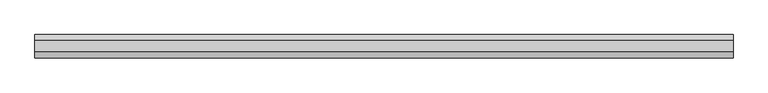
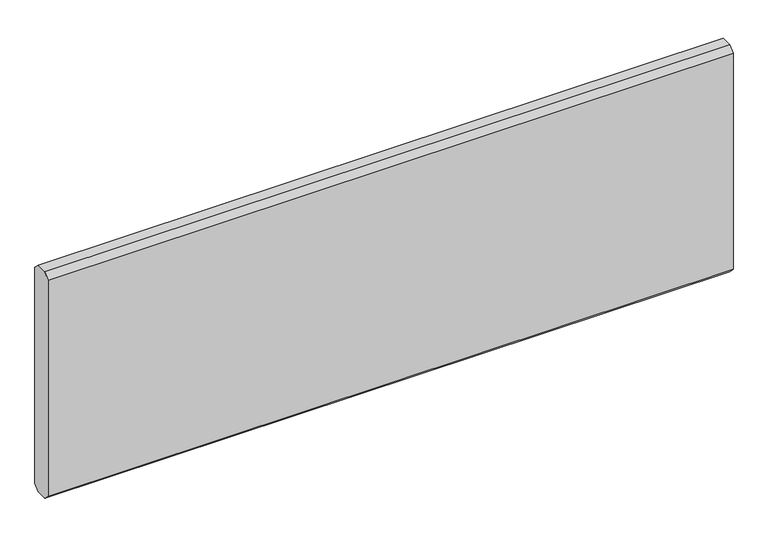
"""IFC4 building model written with IfcOpenShell, lengths in millimetres: proxy geometry, .RIPA : RIPA."""

import ifcopenshell
import ifcopenshell.guid

model = None  # the IFC model being written
_history = None  # IfcOwnerHistory: only IFC2X3 demands one
_inside = {}  # id of a spatial element -> (the spatial element, [elements in it])
_under = {}  # id of a project, library or spatial element -> (it, [spatial elements below it])
_declared = {}  # id of a project -> (the project, [libraries it declares])
_typed = {}  # id of a type object -> (the type object, [elements of that type])
_made_of = {}  # id of a material, layer set ... -> (it, [elements and type objects made of it])


def new_model(schema):
    """Start an empty IFC model of exactly this schema.

    Asked for "IFC4X3", IfcOpenShell would pick the latest addendum, in which some entities
    have other attributes; the version numbers below select the first issue.
    IFC2X3 requires an IfcOwnerHistory on every rooted entity: one is made here for all.
    """
    global model, _history
    if schema == "IFC4X3":
        model = ifcopenshell.file(schema_version=(4, 3, 0, 0))
    else:
        model = ifcopenshell.file(schema=schema)
    _inside.clear()
    _under.clear()
    _declared.clear()
    _typed.clear()
    _made_of.clear()
    _history = None
    if model.schema == "IFC2X3":
        org = make("IfcOrganization", Name="unknown")
        user = make(
            "IfcPersonAndOrganization",
            ThePerson=make("IfcPerson", FamilyName="unknown"),
            TheOrganization=org,
        )
        app = make(
            "IfcApplication",
            ApplicationDeveloper=org,
            Version="unknown",
            ApplicationFullName="unknown",
            ApplicationIdentifier="unknown",
        )
        _history = make(
            "IfcOwnerHistory",
            OwningUser=user,
            OwningApplication=app,
            ChangeAction="ADDED",
            CreationDate=0,
        )
    return model


def make(cls, **values):
    """One entity of the class cls with the attributes given. An attribute that is None is left unset."""
    return model.create_entity(
        cls, **{name: value for name, value in values.items() if value is not None}
    )


def rooted(cls, **values):
    """An entity with a GlobalId (a new one), such as an element, a storey or a relation."""
    return make(cls, GlobalId=ifcopenshell.guid.new(), OwnerHistory=_history, **values)


def si_unit(unit_type, name, prefix=None):
    """IfcSIUnit, for example si_unit("LENGTHUNIT", "METRE", prefix="MILLI")."""
    return make("IfcSIUnit", UnitType=unit_type, Prefix=prefix, Name=name)


def assignment(units):
    """IfcUnitAssignment: the units of a project."""
    return None if units is None else make("IfcUnitAssignment", Units=units)


def point(xyz):
    """IfcCartesianPoint."""
    return None if xyz is None else make("IfcCartesianPoint", Coordinates=xyz)


def direction(xyz):
    """IfcDirection."""
    return None if xyz is None else make("IfcDirection", DirectionRatios=xyz)


def frame(location, z_axis=None, x_axis=None):
    """IfcAxis2Placement3D, a coordinate frame: its origin and axes. An axis left out is left unset."""
    return make(
        "IfcAxis2Placement3D",
        Location=point(location),
        Axis=direction(z_axis),
        RefDirection=direction(x_axis),
    )


def origin():
    """The frame at (0, 0, 0) with its axes left unset."""
    return frame((0.0, 0.0, 0.0))


def place(relative_to, where):
    """IfcLocalPlacement: puts the frame where relative to a parent placement (None: the world)."""
    return make(
        "IfcLocalPlacement", PlacementRelTo=relative_to, RelativePlacement=where
    )


def context(
    kind, dimensions, precision=None, world=None, true_north=None, identifier=None
):
    """IfcGeometricRepresentationContext, for example the 3D "Model" context."""
    return make(
        "IfcGeometricRepresentationContext",
        ContextIdentifier=identifier,
        ContextType=kind,
        CoordinateSpaceDimension=dimensions,
        Precision=precision,
        WorldCoordinateSystem=world,
        TrueNorth=true_north,
    )


def project(units=None, contexts=None):
    """IfcProject with its units and contexts."""
    return rooted(
        "IfcProject",
        Name="project",
        RepresentationContexts=contexts,
        UnitsInContext=assignment(units),
    )


def spatial(cls, under=None, at=None, **own):
    """A site, building, storey or space (cls), placed at a placement, below another one or the project."""
    s = rooted(cls, ObjectPlacement=at, **own)
    if under is not None:
        _under.setdefault(under.id(), (under, []))[1].append(s)
    return s


def polyline(points):
    """IfcPolyline through the points."""
    return make("IfcPolyline", Points=[point(p) for p in points])


def outline(outer, holes=None, kind="AREA"):
    """IfcArbitraryClosedProfileDef: a profile drawn as a closed curve; with holes, ...WithVoids."""
    if holes is None:
        return make("IfcArbitraryClosedProfileDef", ProfileType=kind, OuterCurve=outer)
    return make(
        "IfcArbitraryProfileDefWithVoids",
        ProfileType=kind,
        OuterCurve=outer,
        InnerCurves=holes,
    )


def extrude(swept, where, along, depth):
    """IfcExtrudedAreaSolid: the profile swept, set in the frame where, extruded along a direction by depth."""
    return make(
        "IfcExtrudedAreaSolid",
        SweptArea=swept,
        Position=where,
        ExtrudedDirection=direction(along),
        Depth=depth,
    )


def shape(context_of_items, identifier, shape_type, items):
    """IfcShapeRepresentation: the items that make up one representation, for example the "Body"."""
    return make(
        "IfcShapeRepresentation",
        ContextOfItems=context_of_items,
        RepresentationIdentifier=identifier,
        RepresentationType=shape_type,
        Items=items,
    )


def source(mapping_origin, context_of_items, identifier, shape_type, items):
    """IfcRepresentationMap: a shape defined once, which mapped items show again and again."""
    return make(
        "IfcRepresentationMap",
        MappingOrigin=mapping_origin,
        MappedRepresentation=shape(context_of_items, identifier, shape_type, items),
    )


def transform(
    local_origin,
    x_axis=None,
    y_axis=None,
    z_axis=None,
    scale=None,
    scale2=None,
    scale3=None,
    uniform=True,
):
    """IfcCartesianTransformationOperator3D, or its non-uniform kind. x_axis, y_axis, z_axis: its Axis1, 2, 3."""
    if uniform:
        return make(
            "IfcCartesianTransformationOperator3D",
            Axis1=direction(x_axis),
            Axis2=direction(y_axis),
            LocalOrigin=point(local_origin),
            Scale=scale,
            Axis3=direction(z_axis),
        )
    return make(
        "IfcCartesianTransformationOperator3DnonUniform",
        Axis1=direction(x_axis),
        Axis2=direction(y_axis),
        LocalOrigin=point(local_origin),
        Scale=scale,
        Axis3=direction(z_axis),
        Scale2=scale2,
        Scale3=scale3,
    )


def mapped(mapping_source, mapping_target):
    """IfcMappedItem: shows the shape of a source again, moved by a transform."""
    return make(
        "IfcMappedItem", MappingSource=mapping_source, MappingTarget=mapping_target
    )


def made_of(thing, what):
    """Note that an element or type object is made of a material, layer set ...; save() writes the relation."""
    if what is not None:
        _made_of.setdefault(what.id(), (what, []))[1].append(thing)
    return thing


def element(
    cls,
    number,
    at=None,
    inside=None,
    cuts=None,
    type_object=None,
    material=None,
    context=None,
    identifier="Body",
    shape_type=None,
    held_by="IfcProductDefinitionShape",
    body=None,
    shapes=None,
    **own,
):
    """One element of the class cls, such as IfcWall. Its Tag is "e" and its number.

    at: its placement. inside: the storey or other place that contains it. cuts: it is an
    opening in that element (IfcRelVoidsElement). A single representation is given by context,
    identifier, shape_type and body (its items); several are given by shapes. held_by: the class
    of the entity that holds the representations. save() writes the other relations.
    """
    e = rooted(cls, Tag="e%d" % number, ObjectPlacement=at, **own)
    if body is not None:
        shapes = [shape(context, identifier, shape_type, body)]
    if shapes is not None:
        e.Representation = make(held_by, Representations=shapes)
    if inside is not None:
        _inside.setdefault(inside.id(), (inside, []))[1].append(e)
    if cuts is not None:
        rooted(
            "IfcRelVoidsElement", RelatingBuildingElement=cuts, RelatedOpeningElement=e
        )
    if type_object is not None:
        _typed.setdefault(type_object.id(), (type_object, []))[1].append(e)
    return made_of(e, material)


def aggregate(whole, parts):
    """IfcRelAggregates: a whole, such as a stair, and the parts it consists of."""
    return rooted("IfcRelAggregates", RelatingObject=whole, RelatedObjects=parts)


def save(model, path):
    """Write the relations noted so far, then the file.

    IfcRelAggregates (storeys below a building ...), IfcRelContainedInSpatialStructure (elements
    in a storey), IfcRelDefinesByType, IfcRelAssociatesMaterial and IfcRelDeclares: one each for
    every whole, place, type object, material and project.
    """
    for whole, parts in _under.values():
        aggregate(whole, parts)
    for where, things in _inside.values():
        rooted(
            "IfcRelContainedInSpatialStructure",
            RelatedElements=things,
            RelatingStructure=where,
        )
    for kind, things in _typed.values():
        rooted("IfcRelDefinesByType", RelatedObjects=things, RelatingType=kind)
    for what, things in _made_of.values():
        rooted("IfcRelAssociatesMaterial", RelatedObjects=things, RelatingMaterial=what)
    for by, libraries in _declared.values():
        rooted("IfcRelDeclares", RelatingContext=by, RelatedDefinitions=libraries)
    model.write(path)


def generic_models_d855a693(model_context):
    return source(origin(), model_context, "Body", "SweptSolid", [
        extrude(outline(polyline([(-12.5, 525.0), (12.5, 525.0), (25.0, 512.5), (25.0, 12.5), (12.5, 0.0), (-12.5, 0.0), (-25.0, 12.5), (-25.0, 512.5), (-12.5, 525.0)])), frame((-750.0, 0.0, 0.0), z_axis=(1.0, 0.0, 0.0), x_axis=(0.0, 1.0, 0.0)), (0.0, 0.0, 1.0), 1500.0),
    ])


if __name__ == "__main__":
    model = new_model("IFC4")
    model_context = context("Model", 3, world=origin())
    ifc_project = project(units=[si_unit("LENGTHUNIT", "METRE", prefix="MILLI")], contexts=[model_context])
    site = spatial("IfcSite", under=ifc_project)
    building = spatial("IfcBuilding", under=site)
    placement = place(None, origin())
    generic_models_shape = generic_models_d855a693(model_context)
    element("IfcBuildingElementProxy", 1, Name=".RIPA : RIPA", ObjectType=".RIPA : RIPA", at=placement, inside=building, context=model_context, shape_type="MappedRepresentation", body=[
        mapped(generic_models_shape, transform((0.0, 0.0, 0.0), x_axis=(1.0, 0.0, 0.0), y_axis=(0.0, 1.0, 0.0), z_axis=(0.0, 0.0, 1.0))),
    ])
    save(model, "model.ifc")

# Revit data of these elements
# Type ".RIPA : RIPA"
#   Ripa_largura [instance default] = 0.30 m
#   Ripa_espessura [instance default] = 0.025 m
#   Ripa_comprimento [instance default] = 0.80 m
#   Ripa_chanfo [instance default] = 0.00625 m
#   Ripa_material [instance default] = none
# Element 1 (IfcBuildingElementProxy, ".RIPA : RIPA")
#   Ripa_largura = 0.525 m
#   Ripa_espessura = 0.05 m
#   Ripa_comprimento = 1.50 m
#   Ripa_chanfo = 0.0125 m
#   Ripa_material = .MADEIRA_CEREJEIRA CLARO
#   Materials on its faces: ".MADEIRA_CEREJEIRA CLARO"
# Materials
#   ".MADEIRA_CEREJEIRA CLARO": class ".CC_MADEIRA REVEST.", colour RGB 233 182 144, transparency 0, Cost = 0
